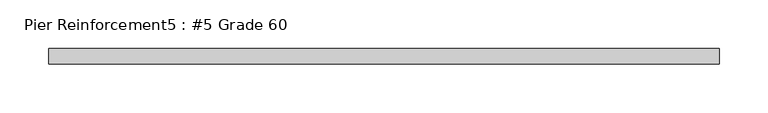
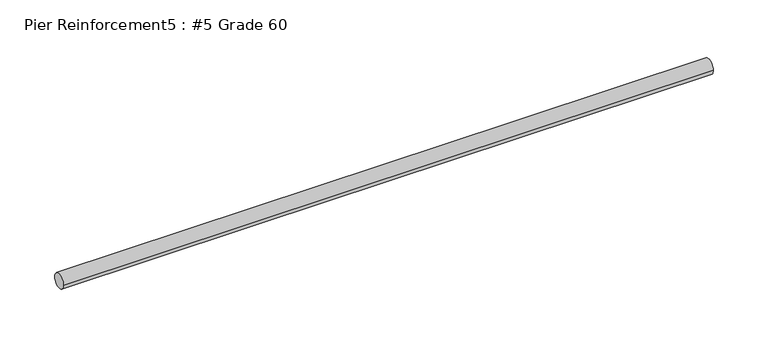
"""IFC4 building model written with IfcOpenShell, lengths in millimetres: proxy geometry, Pier Reinforcement5 : #5 Grade 60."""

from ifc_helpers import new_model, si_unit, point, frame, frame_2d, origin, place, context, project, spatial, circle_curve, trimmed, segment, composite_curve, outline, extrude, source, transform, mapped, element, save


def pier_reinforcement5_5_grade_60_586069a3(model_context):
    return source(origin(), model_context, "Body", "SweptSolid", [
        extrude(outline(composite_curve([segment(trimmed(circle_curve(frame_2d((-534096.6663841, -55.5625)), 7.9375), [point((-534088.7288841, -55.5625))], [point((-534104.6038841, -55.5625))], False, "CARTESIAN"), True, "CONTINUOUS"), segment(trimmed(circle_curve(frame_2d((-534096.6663841, -55.5625)), 7.9375), [point((-534104.6038841, -55.5625))], [point((-534088.7288841, -55.5625))], False, "CARTESIAN"), True, "CONTINUOUS")], self_intersect=False)), frame((589548.1922365, 0.0, 0.0), z_axis=(1.0, 0.0, 0.0), x_axis=(0.0, 1.0, 0.0)), (0.0, 0.0, 1.0), 685.8),
    ])


if __name__ == "__main__":
    model = new_model("IFC4")
    model_context = context("Model", 3, world=origin())
    ifc_project = project(units=[si_unit("LENGTHUNIT", "METRE", prefix="MILLI")], contexts=[model_context])
    site = spatial("IfcSite", under=ifc_project)
    building = spatial("IfcBuilding", under=site)
    placement = place(None, origin())
    pier_reinforcement5_5_grade_60_shape = pier_reinforcement5_5_grade_60_586069a3(model_context)
    element("IfcBuildingElementProxy", 1, Name="Pier Reinforcement5 : #5 Grade 60", ObjectType="Pier Reinforcement5 : #5 Grade 60", at=placement, inside=building, context=model_context, shape_type="MappedRepresentation", body=[
        mapped(pier_reinforcement5_5_grade_60_shape, transform((0.0, 0.0, 0.0), x_axis=(1.0, 0.0, 0.0), y_axis=(0.0, 1.0, 0.0), z_axis=(0.0, 0.0, 1.0))),
    ])
    save(model, "model.ifc")

# Revit data of these elements
# Element 1 (IfcBuildingElementProxy, "Pier Reinforcement5 : #5 Grade 60")
#   Materials on its faces: "#4 GR. 60 REINF. @ 16\" O.C. EW."
# Materials
#   "#4 GR. 60 REINF. @ 16\" O.C. EW.": class "Generic", colour RGB 84 83 81, transparency 0, Cost = 0
